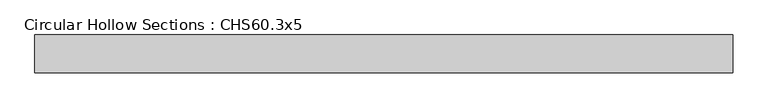
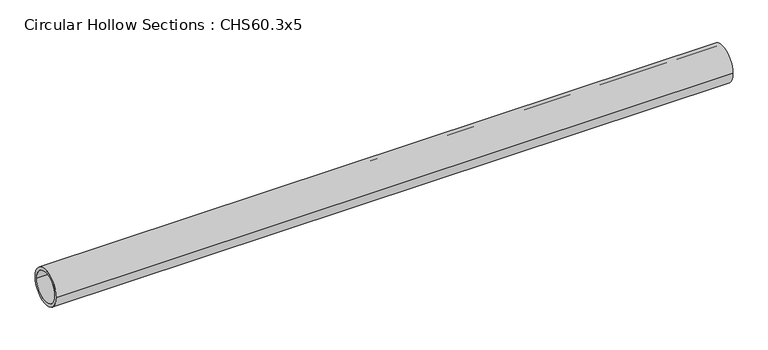
"""IFC4 building model written with IfcOpenShell, lengths in millimetres: beam geometry, Circular Hollow Sections : CHS60.3x5."""

from ifc_helpers import new_model, si_unit, point, frame, origin, origin_2d, place, context, project, spatial, circle_curve, trimmed, segment, composite_curve, outline, extrude, source, transform, mapped, element, save


def circular_hollow_sections_chs60_3x5_c94bd862(model_context):
    return source(origin(), model_context, "Body", "SweptSolid", [
        extrude(outline(composite_curve([segment(trimmed(circle_curve(origin_2d(), 30.15), [point((-30.15, 0.0))], [point((30.15, 0.0))], False, "CARTESIAN"), True, "CONTINUOUS"), segment(trimmed(circle_curve(origin_2d(), 30.15), [point((30.15, 0.0))], [point((-30.15, 0.0))], False, "CARTESIAN"), True, "CONTINUOUS")], self_intersect=False), holes=[composite_curve([segment(trimmed(circle_curve(origin_2d(), 25.15), [point((25.15, 0.0))], [point((-25.15, 0.0))], True, "CARTESIAN"), True, "CONTINUOUS"), segment(trimmed(circle_curve(origin_2d(), 25.15), [point((-25.15, 0.0))], [point((25.15, 0.0))], True, "CARTESIAN"), True, "CONTINUOUS")], self_intersect=False)]), frame((-557.0, 0.0, 0.0), z_axis=(1.0, 0.0, 0.0), x_axis=(0.0, 1.0, 0.0)), (0.0, 0.0, 1.0), 1114.0),
    ])


if __name__ == "__main__":
    model = new_model("IFC4")
    model_context = context("Model", 3, world=origin())
    ifc_project = project(units=[si_unit("LENGTHUNIT", "METRE", prefix="MILLI")], contexts=[model_context])
    site = spatial("IfcSite", under=ifc_project)
    building = spatial("IfcBuilding", under=site)
    placement = place(None, origin())
    circular_hollow_sections_chs60_3x5_shape = circular_hollow_sections_chs60_3x5_c94bd862(model_context)
    element("IfcBeam", 1, ObjectType="Circular Hollow Sections : CHS60.3x5", at=placement, inside=building, context=model_context, shape_type="MappedRepresentation", body=[
        mapped(circular_hollow_sections_chs60_3x5_shape, transform((0.0, 0.0, 0.0), x_axis=(1.0, 0.0, 0.0), y_axis=(0.0, 1.0, 0.0), z_axis=(0.0, 0.0, 1.0))),
    ])
    save(model, "model.ifc")

# Revit data of these elements
# Type "Circular Hollow Sections : CHS60.3x5"
#   Description = "Hollow Core Steel Roof Truss Member"
#   Type Comments = "Steel 50-355"
#   Assembly Code = "F10"
#   t = 5 mm
#   W = 0.00682
#   Start Extension Calculation [instance default] = 3000 mm
#   Start Extension [instance default] = -12.7 mm
#   Length [instance default] = 1500 mm
#   OD = 60.3 mm
#   End Extension Calculation [instance default] = 3000 mm
#   End Extension [instance default] = -12.7 mm
#   A = 0.000869 m²
#   Structural Material [instance default] = Metal - Steel 50-355
# Element 1 (IfcBeam, "Circular Hollow Sections : CHS60.3x5")
#   Materials on its faces: "Metal - Steel 50-355"
# Materials
#   "Metal - Steel 50-355": class "Metal", colour RGB 247 247 247, transparency 0
